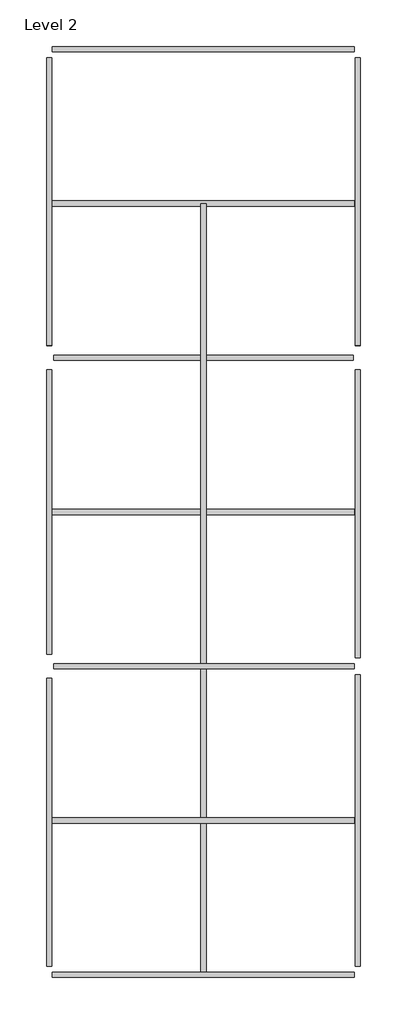
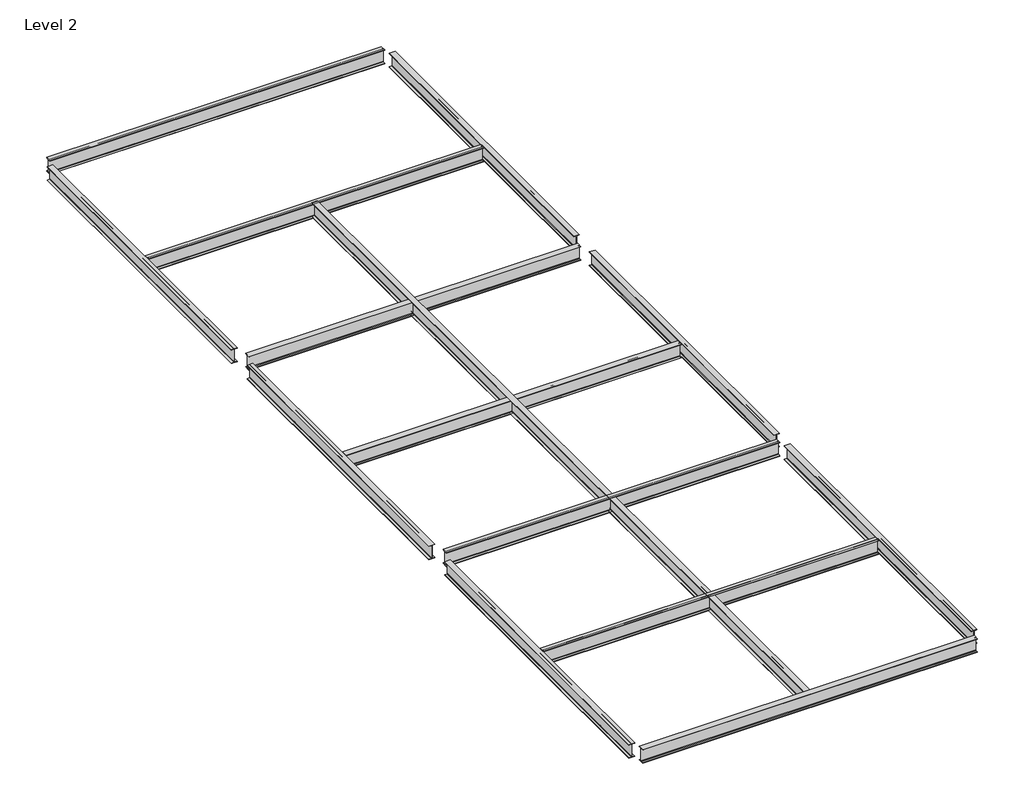
# One storey: 14 beams.
"""IFC4 building model written with IfcOpenShell, lengths in millimetres."""

import ifcopenshell
import ifcopenshell.guid

model = None  # the IFC model being written
_history = None  # IfcOwnerHistory: only IFC2X3 demands one
_inside = {}  # id of a spatial element -> (the spatial element, [elements in it])
_under = {}  # id of a project, library or spatial element -> (it, [spatial elements below it])
_declared = {}  # id of a project -> (the project, [libraries it declares])
_typed = {}  # id of a type object -> (the type object, [elements of that type])
_made_of = {}  # id of a material, layer set ... -> (it, [elements and type objects made of it])


def new_model(schema):
    """Start an empty IFC model of exactly this schema.

    Asked for "IFC4X3", IfcOpenShell would pick the latest addendum, in which some entities
    have other attributes; the version numbers below select the first issue.
    IFC2X3 requires an IfcOwnerHistory on every rooted entity: one is made here for all.
    """
    global model, _history
    if schema == "IFC4X3":
        model = ifcopenshell.file(schema_version=(4, 3, 0, 0))
    else:
        model = ifcopenshell.file(schema=schema)
    _inside.clear()
    _under.clear()
    _declared.clear()
    _typed.clear()
    _made_of.clear()
    _history = None
    if model.schema == "IFC2X3":
        org = make("IfcOrganization", Name="unknown")
        user = make(
            "IfcPersonAndOrganization",
            ThePerson=make("IfcPerson", FamilyName="unknown"),
            TheOrganization=org,
        )
        app = make(
            "IfcApplication",
            ApplicationDeveloper=org,
            Version="unknown",
            ApplicationFullName="unknown",
            ApplicationIdentifier="unknown",
        )
        _history = make(
            "IfcOwnerHistory",
            OwningUser=user,
            OwningApplication=app,
            ChangeAction="ADDED",
            CreationDate=0,
        )
    return model


def make(cls, **values):
    """One entity of the class cls with the attributes given. An attribute that is None is left unset."""
    return model.create_entity(
        cls, **{name: value for name, value in values.items() if value is not None}
    )


def rooted(cls, **values):
    """An entity with a GlobalId (a new one), such as an element, a storey or a relation."""
    return make(cls, GlobalId=ifcopenshell.guid.new(), OwnerHistory=_history, **values)


def si_unit(unit_type, name, prefix=None):
    """IfcSIUnit, for example si_unit("LENGTHUNIT", "METRE", prefix="MILLI")."""
    return make("IfcSIUnit", UnitType=unit_type, Prefix=prefix, Name=name)


def assignment(units):
    """IfcUnitAssignment: the units of a project."""
    return None if units is None else make("IfcUnitAssignment", Units=units)


def point(xyz):
    """IfcCartesianPoint."""
    return None if xyz is None else make("IfcCartesianPoint", Coordinates=xyz)


def direction(xyz):
    """IfcDirection."""
    return None if xyz is None else make("IfcDirection", DirectionRatios=xyz)


def frame(location, z_axis=None, x_axis=None):
    """IfcAxis2Placement3D, a coordinate frame: its origin and axes. An axis left out is left unset."""
    return make(
        "IfcAxis2Placement3D",
        Location=point(location),
        Axis=direction(z_axis),
        RefDirection=direction(x_axis),
    )


def frame_2d(location, x_axis=None):
    """IfcAxis2Placement2D, a coordinate frame in the plane: its origin and x axis."""
    return make(
        "IfcAxis2Placement2D", Location=point(location), RefDirection=direction(x_axis)
    )


def origin():
    """The frame at (0, 0, 0) with its axes left unset."""
    return frame((0.0, 0.0, 0.0))


def place(relative_to, where):
    """IfcLocalPlacement: puts the frame where relative to a parent placement (None: the world)."""
    return make(
        "IfcLocalPlacement", PlacementRelTo=relative_to, RelativePlacement=where
    )


def context(
    kind, dimensions, precision=None, world=None, true_north=None, identifier=None
):
    """IfcGeometricRepresentationContext, for example the 3D "Model" context."""
    return make(
        "IfcGeometricRepresentationContext",
        ContextIdentifier=identifier,
        ContextType=kind,
        CoordinateSpaceDimension=dimensions,
        Precision=precision,
        WorldCoordinateSystem=world,
        TrueNorth=true_north,
    )


def project(units=None, contexts=None):
    """IfcProject with its units and contexts."""
    return rooted(
        "IfcProject",
        Name="project",
        RepresentationContexts=contexts,
        UnitsInContext=assignment(units),
    )


def spatial(cls, under=None, at=None, **own):
    """A site, building, storey or space (cls), placed at a placement, below another one or the project."""
    s = rooted(cls, ObjectPlacement=at, **own)
    if under is not None:
        _under.setdefault(under.id(), (under, []))[1].append(s)
    return s


def polyline(points):
    """IfcPolyline through the points."""
    return make("IfcPolyline", Points=[point(p) for p in points])


def circle_curve(where, radius):
    """IfcCircle in the frame where."""
    return make("IfcCircle", Position=where, Radius=radius)


def trimmed(basis, trim1, trim2, sense, master):
    """IfcTrimmedCurve: the piece of a basis curve between two trims."""
    return make(
        "IfcTrimmedCurve",
        BasisCurve=basis,
        Trim1=trim1,
        Trim2=trim2,
        SenseAgreement=sense,
        MasterRepresentation=master,
    )


def segment(curve, same_sense, transition):
    """IfcCompositeCurveSegment."""
    return make(
        "IfcCompositeCurveSegment",
        Transition=transition,
        SameSense=same_sense,
        ParentCurve=curve,
    )


def composite_curve(segments, self_intersect=None):
    """IfcCompositeCurve: segments joined end to end."""
    return make("IfcCompositeCurve", Segments=segments, SelfIntersect=self_intersect)


def outline(outer, holes=None, kind="AREA"):
    """IfcArbitraryClosedProfileDef: a profile drawn as a closed curve; with holes, ...WithVoids."""
    if holes is None:
        return make("IfcArbitraryClosedProfileDef", ProfileType=kind, OuterCurve=outer)
    return make(
        "IfcArbitraryProfileDefWithVoids",
        ProfileType=kind,
        OuterCurve=outer,
        InnerCurves=holes,
    )


def extrude(swept, where, along, depth):
    """IfcExtrudedAreaSolid: the profile swept, set in the frame where, extruded along a direction by depth."""
    return make(
        "IfcExtrudedAreaSolid",
        SweptArea=swept,
        Position=where,
        ExtrudedDirection=direction(along),
        Depth=depth,
    )


def shape(context_of_items, identifier, shape_type, items):
    """IfcShapeRepresentation: the items that make up one representation, for example the "Body"."""
    return make(
        "IfcShapeRepresentation",
        ContextOfItems=context_of_items,
        RepresentationIdentifier=identifier,
        RepresentationType=shape_type,
        Items=items,
    )


def source(mapping_origin, context_of_items, identifier, shape_type, items):
    """IfcRepresentationMap: a shape defined once, which mapped items show again and again."""
    return make(
        "IfcRepresentationMap",
        MappingOrigin=mapping_origin,
        MappedRepresentation=shape(context_of_items, identifier, shape_type, items),
    )


def transform(
    local_origin,
    x_axis=None,
    y_axis=None,
    z_axis=None,
    scale=None,
    scale2=None,
    scale3=None,
    uniform=True,
):
    """IfcCartesianTransformationOperator3D, or its non-uniform kind. x_axis, y_axis, z_axis: its Axis1, 2, 3."""
    if uniform:
        return make(
            "IfcCartesianTransformationOperator3D",
            Axis1=direction(x_axis),
            Axis2=direction(y_axis),
            LocalOrigin=point(local_origin),
            Scale=scale,
            Axis3=direction(z_axis),
        )
    return make(
        "IfcCartesianTransformationOperator3DnonUniform",
        Axis1=direction(x_axis),
        Axis2=direction(y_axis),
        LocalOrigin=point(local_origin),
        Scale=scale,
        Axis3=direction(z_axis),
        Scale2=scale2,
        Scale3=scale3,
    )


def mapped(mapping_source, mapping_target):
    """IfcMappedItem: shows the shape of a source again, moved by a transform."""
    return make(
        "IfcMappedItem", MappingSource=mapping_source, MappingTarget=mapping_target
    )


def made_of(thing, what):
    """Note that an element or type object is made of a material, layer set ...; save() writes the relation."""
    if what is not None:
        _made_of.setdefault(what.id(), (what, []))[1].append(thing)
    return thing


def element(
    cls,
    number,
    at=None,
    inside=None,
    cuts=None,
    type_object=None,
    material=None,
    context=None,
    identifier="Body",
    shape_type=None,
    held_by="IfcProductDefinitionShape",
    body=None,
    shapes=None,
    **own,
):
    """One element of the class cls, such as IfcWall. Its Tag is "e" and its number.

    at: its placement. inside: the storey or other place that contains it. cuts: it is an
    opening in that element (IfcRelVoidsElement). A single representation is given by context,
    identifier, shape_type and body (its items); several are given by shapes. held_by: the class
    of the entity that holds the representations. save() writes the other relations.
    """
    e = rooted(cls, Tag="e%d" % number, ObjectPlacement=at, **own)
    if body is not None:
        shapes = [shape(context, identifier, shape_type, body)]
    if shapes is not None:
        e.Representation = make(held_by, Representations=shapes)
    if inside is not None:
        _inside.setdefault(inside.id(), (inside, []))[1].append(e)
    if cuts is not None:
        rooted(
            "IfcRelVoidsElement", RelatingBuildingElement=cuts, RelatedOpeningElement=e
        )
    if type_object is not None:
        _typed.setdefault(type_object.id(), (type_object, []))[1].append(e)
    return made_of(e, material)


def aggregate(whole, parts):
    """IfcRelAggregates: a whole, such as a stair, and the parts it consists of."""
    return rooted("IfcRelAggregates", RelatingObject=whole, RelatedObjects=parts)


def save(model, path):
    """Write the relations noted so far, then the file.

    IfcRelAggregates (storeys below a building ...), IfcRelContainedInSpatialStructure (elements
    in a storey), IfcRelDefinesByType, IfcRelAssociatesMaterial and IfcRelDeclares: one each for
    every whole, place, type object, material and project.
    """
    for whole, parts in _under.values():
        aggregate(whole, parts)
    for where, things in _inside.values():
        rooted(
            "IfcRelContainedInSpatialStructure",
            RelatedElements=things,
            RelatingStructure=where,
        )
    for kind, things in _typed.values():
        rooted("IfcRelDefinesByType", RelatedObjects=things, RelatingType=kind)
    for what, things in _made_of.values():
        rooted("IfcRelAssociatesMaterial", RelatedObjects=things, RelatingMaterial=what)
    for by, libraries in _declared.values():
        rooted("IfcRelDeclares", RelatingContext=by, RelatedDefinitions=libraries)
    model.write(path)


def ub_universal_beams_ub254x102x22_5313c1c2(model_context):
    return source(origin(), model_context, "Body", "SweptSolid", [
        extrude(outline(composite_curve([segment(polyline([(50.8, -120.2), (50.8, -127.0), (-50.8, -127.0), (-50.8, -120.2), (-10.45, -120.2)]), True, "CONTINUOUS"), segment(trimmed(circle_curve(frame_2d((-10.45, -112.6)), 7.6), [point((-10.45, -120.2))], [point((-2.85, -112.6))], True, "CARTESIAN"), True, "CONTINUOUS"), segment(polyline([(-2.85, -112.6), (-2.85, 112.6)]), True, "CONTINUOUS"), segment(trimmed(circle_curve(frame_2d((-10.45, 112.6)), 7.6), [point((-2.85, 112.6))], [point((-10.45, 120.2))], True, "CARTESIAN"), True, "CONTINUOUS"), segment(polyline([(-10.45, 120.2), (-50.8, 120.2), (-50.8, 127.0), (50.8, 127.0), (50.8, 120.2), (10.45, 120.2)]), True, "CONTINUOUS"), segment(trimmed(circle_curve(frame_2d((10.45, 112.6)), 7.6), [point((10.45, 120.2))], [point((2.85, 112.6))], True, "CARTESIAN"), True, "CONTINUOUS"), segment(polyline([(2.85, 112.6), (2.85, -112.6)]), True, "CONTINUOUS"), segment(trimmed(circle_curve(frame_2d((10.45, -112.6)), 7.6), [point((2.85, -112.6))], [point((10.45, -120.2))], True, "CARTESIAN"), True, "CONTINUOUS"), segment(polyline([(10.45, -120.2), (50.8, -120.2)]), True, "CONTINUOUS")], self_intersect=False)), frame((-2834.7, 0.0, 0.0), z_axis=(1.0, 0.0, 0.0), x_axis=(0.0, 1.0, 0.0)), (0.0, 0.0, 1.0), 5597.1),
    ])


def ub_universal_beams_ub254x102x22_9642d6a0(model_context):
    return source(origin(), model_context, "Body", "SweptSolid", [
        extrude(outline(composite_curve([segment(polyline([(50.8, -120.2), (50.8, -127.0), (-50.8, -127.0), (-50.8, -120.2), (-10.45, -120.2)]), True, "CONTINUOUS"), segment(trimmed(circle_curve(frame_2d((-10.45, -112.6)), 7.6), [point((-10.45, -120.2))], [point((-2.85, -112.6))], True, "CARTESIAN"), True, "CONTINUOUS"), segment(polyline([(-2.85, -112.6), (-2.85, 112.6)]), True, "CONTINUOUS"), segment(trimmed(circle_curve(frame_2d((-10.45, 112.6)), 7.6), [point((-2.85, 112.6))], [point((-10.45, 120.2))], True, "CARTESIAN"), True, "CONTINUOUS"), segment(polyline([(-10.45, 120.2), (-50.8, 120.2), (-50.8, 127.0), (50.8, 127.0), (50.8, 120.2), (10.45, 120.2)]), True, "CONTINUOUS"), segment(trimmed(circle_curve(frame_2d((10.45, 112.6)), 7.6), [point((10.45, 120.2))], [point((2.85, 112.6))], True, "CARTESIAN"), True, "CONTINUOUS"), segment(polyline([(2.85, 112.6), (2.85, -112.6)]), True, "CONTINUOUS"), segment(trimmed(circle_curve(frame_2d((10.45, -112.6)), 7.6), [point((2.85, -112.6))], [point((10.45, -120.2))], True, "CARTESIAN"), True, "CONTINUOUS"), segment(polyline([(10.45, -120.2), (50.8, -120.2)]), True, "CONTINUOUS")], self_intersect=False)), frame((-2762.4, 0.0, 0.0), z_axis=(1.0, 0.0, 0.0), x_axis=(0.0, 1.0, 0.0)), (0.0, 0.0, 1.0), 5524.8),
    ])


def ub_universal_beams_ub254x102x22_6668b1ee(model_context):
    return source(origin(), model_context, "Body", "SweptSolid", [
        extrude(outline(composite_curve([segment(polyline([(50.8, -120.2), (50.8, -127.0), (-50.8, -127.0), (-50.8, -120.2), (-10.45, -120.2)]), True, "CONTINUOUS"), segment(trimmed(circle_curve(frame_2d((-10.45, -112.6)), 7.6), [point((-10.45, -120.2))], [point((-2.85, -112.6))], True, "CARTESIAN"), True, "CONTINUOUS"), segment(polyline([(-2.85, -112.6), (-2.85, 112.6)]), True, "CONTINUOUS"), segment(trimmed(circle_curve(frame_2d((-10.45, 112.6)), 7.6), [point((-2.85, 112.6))], [point((-10.45, 120.2))], True, "CARTESIAN"), True, "CONTINUOUS"), segment(polyline([(-10.45, 120.2), (-50.8, 120.2), (-50.8, 127.0), (50.8, 127.0), (50.8, 120.2), (10.45, 120.2)]), True, "CONTINUOUS"), segment(trimmed(circle_curve(frame_2d((10.45, 112.6)), 7.6), [point((10.45, 120.2))], [point((2.85, 112.6))], True, "CARTESIAN"), True, "CONTINUOUS"), segment(polyline([(2.85, 112.6), (2.85, -112.6)]), True, "CONTINUOUS"), segment(trimmed(circle_curve(frame_2d((10.45, -112.6)), 7.6), [point((2.85, -112.6))], [point((10.45, -120.2))], True, "CARTESIAN"), True, "CONTINUOUS"), segment(polyline([(10.45, -120.2), (50.8, -120.2)]), True, "CONTINUOUS")], self_intersect=False)), frame((-2762.4, 0.0, 0.0), z_axis=(1.0, 0.0, 0.0), x_axis=(0.0, 1.0, 0.0)), (0.0, 0.0, 1.0), 5597.1),
    ])


def ub_universal_beams_ub254x102x22_dcacaae8(model_context):
    return source(origin(), model_context, "Body", "SweptSolid", [
        extrude(outline(composite_curve([segment(polyline([(50.8, -120.2), (50.8, -127.0), (-50.8, -127.0), (-50.8, -120.2), (-10.45, -120.2)]), True, "CONTINUOUS"), segment(trimmed(circle_curve(frame_2d((-10.45, -112.6)), 7.6), [point((-10.45, -120.2))], [point((-2.85, -112.6))], True, "CARTESIAN"), True, "CONTINUOUS"), segment(polyline([(-2.85, -112.6), (-2.85, 112.6)]), True, "CONTINUOUS"), segment(trimmed(circle_curve(frame_2d((-10.45, 112.6)), 7.6), [point((-2.85, 112.6))], [point((-10.45, 120.2))], True, "CARTESIAN"), True, "CONTINUOUS"), segment(polyline([(-10.45, 120.2), (-50.8, 120.2), (-50.8, 127.0), (50.8, 127.0), (50.8, 120.2), (10.45, 120.2)]), True, "CONTINUOUS"), segment(trimmed(circle_curve(frame_2d((10.45, 112.6)), 7.6), [point((10.45, 120.2))], [point((2.85, 112.6))], True, "CARTESIAN"), True, "CONTINUOUS"), segment(polyline([(2.85, 112.6), (2.85, -112.6)]), True, "CONTINUOUS"), segment(trimmed(circle_curve(frame_2d((10.45, -112.6)), 7.6), [point((2.85, -112.6))], [point((10.45, -120.2))], True, "CARTESIAN"), True, "CONTINUOUS"), segment(polyline([(10.45, -120.2), (50.8, -120.2)]), True, "CONTINUOUS")], self_intersect=False)), frame((-2936.5, 0.0, 0.0), z_axis=(1.0, 0.0, 0.0), x_axis=(0.0, 1.0, 0.0)), (0.0, 0.0, 1.0), 5873.0),
    ])


def ub_universal_beams_ub254x102x22_ea344768(model_context):
    return source(origin(), model_context, "Body", "SweptSolid", [
        extrude(outline(composite_curve([segment(polyline([(50.8, -120.2), (50.8, -127.0), (-50.8, -127.0), (-50.8, -120.2), (-10.45, -120.2)]), True, "CONTINUOUS"), segment(trimmed(circle_curve(frame_2d((-10.45, -112.6)), 7.6), [point((-10.45, -120.2))], [point((-2.85, -112.6))], True, "CARTESIAN"), True, "CONTINUOUS"), segment(polyline([(-2.85, -112.6), (-2.85, 112.6)]), True, "CONTINUOUS"), segment(trimmed(circle_curve(frame_2d((-10.45, 112.6)), 7.6), [point((-2.85, 112.6))], [point((-10.45, 120.2))], True, "CARTESIAN"), True, "CONTINUOUS"), segment(polyline([(-10.45, 120.2), (-50.8, 120.2), (-50.8, 127.0), (50.8, 127.0), (50.8, 120.2), (10.45, 120.2)]), True, "CONTINUOUS"), segment(trimmed(circle_curve(frame_2d((10.45, 112.6)), 7.6), [point((10.45, 120.2))], [point((2.85, 112.6))], True, "CARTESIAN"), True, "CONTINUOUS"), segment(polyline([(2.85, 112.6), (2.85, -112.6)]), True, "CONTINUOUS"), segment(trimmed(circle_curve(frame_2d((10.45, -112.6)), 7.6), [point((2.85, -112.6))], [point((10.45, -120.2))], True, "CARTESIAN"), True, "CONTINUOUS"), segment(polyline([(10.45, -120.2), (50.8, -120.2)]), True, "CONTINUOUS")], self_intersect=False)), frame((-2911.1, 0.0, 0.0), z_axis=(1.0, 0.0, 0.0), x_axis=(0.0, 1.0, 0.0)), (0.0, 0.0, 1.0), 5822.2),
    ])


def ub_universal_beams_ub254x102x22_fd37447c(model_context):
    return source(origin(), model_context, "Body", "SweptSolid", [
        extrude(outline(composite_curve([segment(polyline([(50.8, -120.2), (50.8, -127.0), (-50.8, -127.0), (-50.8, -120.2), (-10.45, -120.2)]), True, "CONTINUOUS"), segment(trimmed(circle_curve(frame_2d((-10.45, -112.6)), 7.6), [point((-10.45, -120.2))], [point((-2.85, -112.6))], True, "CARTESIAN"), True, "CONTINUOUS"), segment(polyline([(-2.85, -112.6), (-2.85, 112.6)]), True, "CONTINUOUS"), segment(trimmed(circle_curve(frame_2d((-10.45, 112.6)), 7.6), [point((-2.85, 112.6))], [point((-10.45, 120.2))], True, "CARTESIAN"), True, "CONTINUOUS"), segment(polyline([(-10.45, 120.2), (-50.8, 120.2), (-50.8, 127.0), (50.8, 127.0), (50.8, 120.2), (10.45, 120.2)]), True, "CONTINUOUS"), segment(trimmed(circle_curve(frame_2d((10.45, 112.6)), 7.6), [point((10.45, 120.2))], [point((2.85, 112.6))], True, "CARTESIAN"), True, "CONTINUOUS"), segment(polyline([(2.85, 112.6), (2.85, -112.6)]), True, "CONTINUOUS"), segment(trimmed(circle_curve(frame_2d((10.45, -112.6)), 7.6), [point((2.85, -112.6))], [point((10.45, -120.2))], True, "CARTESIAN"), True, "CONTINUOUS"), segment(polyline([(10.45, -120.2), (50.8, -120.2)]), True, "CONTINUOUS")], self_intersect=False)), frame((-2834.7, 0.0, 0.0), z_axis=(1.0, 0.0, 0.0), x_axis=(0.0, 1.0, 0.0)), (0.0, 0.0, 1.0), 5669.4),
    ])


def ub_universal_beams_ub254x102x22_c294fd8a(model_context):
    return source(origin(), model_context, "Body", "SweptSolid", [
        extrude(outline(composite_curve([segment(polyline([(50.8, -120.2), (50.8, -127.0), (-50.8, -127.0), (-50.8, -120.2), (-10.45, -120.2)]), True, "CONTINUOUS"), segment(trimmed(circle_curve(frame_2d((-10.45, -112.6)), 7.6), [point((-10.45, -120.2))], [point((-2.85, -112.6))], True, "CARTESIAN"), True, "CONTINUOUS"), segment(polyline([(-2.85, -112.6), (-2.85, 112.6)]), True, "CONTINUOUS"), segment(trimmed(circle_curve(frame_2d((-10.45, 112.6)), 7.6), [point((-2.85, 112.6))], [point((-10.45, 120.2))], True, "CARTESIAN"), True, "CONTINUOUS"), segment(polyline([(-10.45, 120.2), (-50.8, 120.2), (-50.8, 127.0), (50.8, 127.0), (50.8, 120.2), (10.45, 120.2)]), True, "CONTINUOUS"), segment(trimmed(circle_curve(frame_2d((10.45, 112.6)), 7.6), [point((10.45, 120.2))], [point((2.85, 112.6))], True, "CARTESIAN"), True, "CONTINUOUS"), segment(polyline([(2.85, 112.6), (2.85, -112.6)]), True, "CONTINUOUS"), segment(trimmed(circle_curve(frame_2d((10.45, -112.6)), 7.6), [point((2.85, -112.6))], [point((10.45, -120.2))], True, "CARTESIAN"), True, "CONTINUOUS"), segment(polyline([(10.45, -120.2), (50.8, -120.2)]), True, "CONTINUOUS")], self_intersect=False)), frame((-2936.5, 0.0, 0.0), z_axis=(1.0, 0.0, 0.0), x_axis=(0.0, 1.0, 0.0)), (0.0, 0.0, 1.0), 5847.6),
    ])


def ub_universal_beams_ub254x102x22_297c9696(model_context):
    return source(origin(), model_context, "Body", "SweptSolid", [
        extrude(outline(composite_curve([segment(polyline([(50.8, -120.2), (50.8, -127.0), (-50.8, -127.0), (-50.8, -120.2), (-10.45, -120.2)]), True, "CONTINUOUS"), segment(trimmed(circle_curve(frame_2d((-10.45, -112.6)), 7.6), [point((-10.45, -120.2))], [point((-2.85, -112.6))], True, "CARTESIAN"), True, "CONTINUOUS"), segment(polyline([(-2.85, -112.6), (-2.85, 112.6)]), True, "CONTINUOUS"), segment(trimmed(circle_curve(frame_2d((-10.45, 112.6)), 7.6), [point((-2.85, 112.6))], [point((-10.45, 120.2))], True, "CARTESIAN"), True, "CONTINUOUS"), segment(polyline([(-10.45, 120.2), (-50.8, 120.2), (-50.8, 127.0), (50.8, 127.0), (50.8, 120.2), (10.45, 120.2)]), True, "CONTINUOUS"), segment(trimmed(circle_curve(frame_2d((10.45, 112.6)), 7.6), [point((10.45, 120.2))], [point((2.85, 112.6))], True, "CARTESIAN"), True, "CONTINUOUS"), segment(polyline([(2.85, 112.6), (2.85, -112.6)]), True, "CONTINUOUS"), segment(trimmed(circle_curve(frame_2d((10.45, -112.6)), 7.6), [point((2.85, -112.6))], [point((10.45, -120.2))], True, "CARTESIAN"), True, "CONTINUOUS"), segment(polyline([(10.45, -120.2), (50.8, -120.2)]), True, "CONTINUOUS")], self_intersect=False)), frame((-7349.2, 0.0, 0.0), z_axis=(1.0, 0.0, 0.0), x_axis=(0.0, 1.0, 0.0)), (0.0, 0.0, 1.0), 14946.35),
    ])


model = new_model("IFC4")

# Units and contexts
model_context = context("Model", 3, world=origin())
ifc_project = project(units=[si_unit("LENGTHUNIT", "METRE", prefix="MILLI")], contexts=[model_context])

# Site, building, storey
site = spatial("IfcSite", under=ifc_project)
building = spatial("IfcBuilding", under=site)
storey = spatial("IfcBuildingStorey", under=building, Name="Level 2", Elevation=2000.0)

# Beams
placement = place(None, origin())
ub_universal_beams_ub254x102x22_shape = ub_universal_beams_ub254x102x22_5313c1c2(model_context)
element("IfcBeam", 1, ObjectType="UB-Universal Beams : UB254x102x22", at=placement, inside=storey, context=model_context, shape_type="MappedRepresentation", body=[
    mapped(ub_universal_beams_ub254x102x22_shape, transform((-3383.1518909, -8313.6046839, 1873.0), x_axis=(0.0, 1.0, 0.0), y_axis=(-1.0, 0.0, 0.0), z_axis=(0.0, 0.0, 1.0))),
])
element("IfcBeam", 2, ObjectType="UB-Universal Beams : UB254x102x22", at=placement, inside=storey, context=model_context, shape_type="MappedRepresentation", body=[
    mapped(ub_universal_beams_ub254x102x22_shape, transform((2616.8481091, 3686.3953161, 1873.0), x_axis=(0.0, -1.0, 0.0), y_axis=(1.0, 0.0, 0.0), z_axis=(0.0, 0.0, 1.0))),
])
ub_universal_beams_ub254x102x22_2_shape = ub_universal_beams_ub254x102x22_9642d6a0(model_context)
element("IfcBeam", 3, ObjectType="UB-Universal Beams : UB254x102x22", at=placement, inside=storey, context=model_context, shape_type="MappedRepresentation", body=[
    mapped(ub_universal_beams_ub254x102x22_2_shape, transform((-3383.1518909, -2313.6046839, 1873.0), x_axis=(0.0, 1.0, 0.0), y_axis=(-1.0, 0.0, 0.0), z_axis=(0.0, 0.0, 1.0))),
])
ub_universal_beams_ub254x102x22_3_shape = ub_universal_beams_ub254x102x22_6668b1ee(model_context)
element("IfcBeam", 4, ObjectType="UB-Universal Beams : UB254x102x22", at=placement, inside=storey, context=model_context, shape_type="MappedRepresentation", body=[
    mapped(ub_universal_beams_ub254x102x22_3_shape, transform((-3383.1518909, 3686.3953161, 1873.0), x_axis=(0.0, 1.0, 0.0), y_axis=(-1.0, 0.0, 0.0), z_axis=(0.0, 0.0, 1.0))),
])
element("IfcBeam", 5, ObjectType="UB-Universal Beams : UB254x102x22", at=placement, inside=storey, context=model_context, shape_type="MappedRepresentation", body=[
    mapped(ub_universal_beams_ub254x102x22_3_shape, transform((2616.8481091, -2313.6046839, 1873.0), x_axis=(0.0, -1.0, 0.0), y_axis=(1.0, 0.0, 0.0), z_axis=(0.0, 0.0, 1.0))),
])
ub_universal_beams_ub254x102x22_4_shape = ub_universal_beams_ub254x102x22_dcacaae8(model_context)
element("IfcBeam", 6, ObjectType="UB-Universal Beams : UB254x102x22", at=placement, inside=storey, context=model_context, shape_type="MappedRepresentation", body=[
    mapped(ub_universal_beams_ub254x102x22_4_shape, transform((-383.1518909, 6686.3953161, 1873.0), x_axis=(1.0, 0.0, 0.0), y_axis=(0.0, 1.0, 0.0), z_axis=(0.0, 0.0, 1.0))),
])
element("IfcBeam", 7, ObjectType="UB-Universal Beams : UB254x102x22", at=placement, inside=storey, context=model_context, shape_type="MappedRepresentation", body=[
    mapped(ub_universal_beams_ub254x102x22_4_shape, transform((-383.1518909, -11313.6046839, 1873.0), x_axis=(-1.0, 0.0, 0.0), y_axis=(0.0, -1.0, 0.0), z_axis=(0.0, 0.0, 1.0))),
])
element("IfcBeam", 8, ObjectType="UB-Universal Beams : UB254x102x22", at=placement, inside=storey, context=model_context, shape_type="MappedRepresentation", body=[
    mapped(ub_universal_beams_ub254x102x22_4_shape, transform((-383.1518909, -8313.6046839, 1873.0), x_axis=(1.0, 0.0, 0.0), y_axis=(0.0, 1.0, 0.0), z_axis=(0.0, 0.0, 1.0))),
])
element("IfcBeam", 9, ObjectType="UB-Universal Beams : UB254x102x22", at=placement, inside=storey, context=model_context, shape_type="MappedRepresentation", body=[
    mapped(ub_universal_beams_ub254x102x22_4_shape, transform((-383.1518909, 3686.3953161, 1873.0), x_axis=(1.0, 0.0, 0.0), y_axis=(0.0, 1.0, 0.0), z_axis=(0.0, 0.0, 1.0))),
])
element("IfcBeam", 10, ObjectType="UB-Universal Beams : UB254x102x22", at=placement, inside=storey, context=model_context, shape_type="MappedRepresentation", body=[
    mapped(ub_universal_beams_ub254x102x22_4_shape, transform((-383.1518909, -2313.6046839, 1873.0), x_axis=(1.0, 0.0, 0.0), y_axis=(0.0, 1.0, 0.0), z_axis=(0.0, 0.0, 1.0))),
])
ub_universal_beams_ub254x102x22_5_shape = ub_universal_beams_ub254x102x22_ea344768(model_context)
element("IfcBeam", 11, ObjectType="UB-Universal Beams : UB254x102x22", at=placement, inside=storey, context=model_context, shape_type="MappedRepresentation", body=[
    mapped(ub_universal_beams_ub254x102x22_5_shape, transform((-383.1518909, 686.3953161, 1873.0), x_axis=(-1.0, 0.0, 0.0), y_axis=(0.0, -1.0, 0.0), z_axis=(0.0, 0.0, 1.0))),
])
ub_universal_beams_ub254x102x22_6_shape = ub_universal_beams_ub254x102x22_fd37447c(model_context)
element("IfcBeam", 12, ObjectType="UB-Universal Beams : UB254x102x22", at=placement, inside=storey, context=model_context, shape_type="MappedRepresentation", body=[
    mapped(ub_universal_beams_ub254x102x22_6_shape, transform((2616.8481091, -8313.6046839, 1873.0), x_axis=(0.0, -1.0, 0.0), y_axis=(1.0, 0.0, 0.0), z_axis=(0.0, 0.0, 1.0))),
])
ub_universal_beams_ub254x102x22_7_shape = ub_universal_beams_ub254x102x22_c294fd8a(model_context)
element("IfcBeam", 13, ObjectType="UB-Universal Beams : UB254x102x22", at=placement, inside=storey, context=model_context, shape_type="MappedRepresentation", body=[
    mapped(ub_universal_beams_ub254x102x22_7_shape, transform((-383.1518909, -5313.6046839, 1873.0), x_axis=(-1.0, 0.0, 0.0), y_axis=(0.0, -1.0, 0.0), z_axis=(0.0, 0.0, 1.0))),
])
ub_universal_beams_ub254x102x22_8_shape = ub_universal_beams_ub254x102x22_297c9696(model_context)
element("IfcBeam", 14, ObjectType="UB-Universal Beams : UB254x102x22", at=placement, inside=storey, context=model_context, shape_type="MappedRepresentation", body=[
    mapped(ub_universal_beams_ub254x102x22_8_shape, transform((-383.1518909, -3913.6046839, 1873.0), x_axis=(0.0, 1.0, 0.0), y_axis=(-1.0, 0.0, 0.0), z_axis=(0.0, 0.0, 1.0))),
])

save(model, "model.ifc")

# Revit data of these elements
# Type "UB-Universal Beams : UB254x102x22"
#   Section Name Key = "UB254X102X22"
#   Width = 10.16 cm
#   Web Thickness = 0.57 cm
#   Web Fillet = 0.76 cm
#   Warping Constant = 18200.0 cm⁶
#   Torsional Moment of Inertia = 4.15 cm⁴
#   Section Area = 28.0 cm²
#   Plastic Modulus weak axis = 37.3 cm³
#   Plastic Modulus strong axis = 259.0 cm³
#   Nominal Weight = 22.00 kgf/m
#   Moment of Inertia weak axis = 119.00 cm⁴
#   Moment of Inertia strong axis = 2841.00 cm⁴
#   Height = 25.4 cm
#   Flange Thickness = 0.68 cm
#   Elastic Modulus weak axis = 23.5 cm³
#   Elastic Modulus strong axis = 224.0 cm³
#   Centroid Vertical = 12.7 cm
#   Centroid Horizontal = 5.08 cm
#   Bolt Spacing = 5.4 cm
#   Length [instance default] = 1500 mm
#   Structural Material [instance default] = Metal - Steel 43-275
#   Type Comments = ""
#   Assembly Code = ""
# Elements 1, 2, 3, 4, 5, 6, 7, 8, 9, 10, 11, 12, 13, 14 (IfcBeam, "UB-Universal Beams : UB254x102x22")
#   Structural Material = Metal - Steel 43-275
#   Phase Created = New Construction
#   Materials on its faces: "Metal - Steel 43-275"
# Materials
#   "Metal - Steel 43-275": class "Metal", colour RGB 247 247 247, transparency 0, Cost = 0
